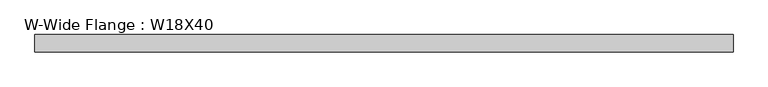
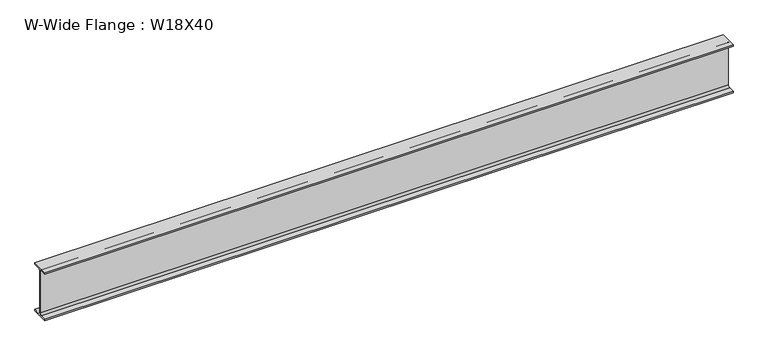
"""IFC4 building model written with IfcOpenShell, lengths in millimetres: beam geometry, W-Wide Flange : W18X40."""

from ifc_helpers import new_model, si_unit, point, frame, frame_2d, origin, place, context, project, spatial, polyline, circle_curve, trimmed, segment, composite_curve, outline, extrude, source, transform, mapped, element, save


def w_wide_flange_w18x40_5b02e5c9(model_context):
    return source(origin(), model_context, "Body", "SweptSolid", [
        extrude(outline(composite_curve([segment(polyline([(76.454, -213.995), (76.454, -227.33), (-76.454, -227.33), (-76.454, -213.995), (-20.828, -213.995)]), True, "CONTINUOUS"), segment(trimmed(circle_curve(frame_2d((-20.828, -197.1675)), 16.8275), [point((-20.828, -213.995))], [point((-4.0005, -197.1675))], True, "CARTESIAN"), True, "CONTINUOUS"), segment(polyline([(-4.0005, -197.1675), (-4.0005, 197.1675)]), True, "CONTINUOUS"), segment(trimmed(circle_curve(frame_2d((-20.828, 197.1675)), 16.8275), [point((-4.0005, 197.1675))], [point((-20.828, 213.995))], True, "CARTESIAN"), True, "CONTINUOUS"), segment(polyline([(-20.828, 213.995), (-76.454, 213.995), (-76.454, 227.33), (76.454, 227.33), (76.454, 213.995), (20.828, 213.995)]), True, "CONTINUOUS"), segment(trimmed(circle_curve(frame_2d((20.828, 197.1675)), 16.8275), [point((20.828, 213.995))], [point((4.0005, 197.1675))], True, "CARTESIAN"), True, "CONTINUOUS"), segment(polyline([(4.0005, 197.1675), (4.0005, -197.1675)]), True, "CONTINUOUS"), segment(trimmed(circle_curve(frame_2d((20.828, -197.1675)), 16.8275), [point((4.0005, -197.1675))], [point((20.828, -213.995))], True, "CARTESIAN"), True, "CONTINUOUS"), segment(polyline([(20.828, -213.995), (76.454, -213.995)]), True, "CONTINUOUS")], self_intersect=False)), frame((-3079.75, 0.0, 0.0), z_axis=(1.0, 0.0, 0.0), x_axis=(0.0, 1.0, 0.0)), (0.0, 0.0, 1.0), 6159.5),
    ])


if __name__ == "__main__":
    model = new_model("IFC4")
    model_context = context("Model", 3, world=origin())
    ifc_project = project(units=[si_unit("LENGTHUNIT", "METRE", prefix="MILLI")], contexts=[model_context])
    site = spatial("IfcSite", under=ifc_project)
    building = spatial("IfcBuilding", under=site)
    placement = place(None, origin())
    w_wide_flange_w18x40_shape = w_wide_flange_w18x40_5b02e5c9(model_context)
    element("IfcBeam", 1, ObjectType="W-Wide Flange : W18X40", at=placement, inside=building, context=model_context, shape_type="MappedRepresentation", body=[
        mapped(w_wide_flange_w18x40_shape, transform((0.0, 0.0, 0.0), x_axis=(1.0, 0.0, 0.0), y_axis=(0.0, 1.0, 0.0), z_axis=(0.0, 0.0, 1.0))),
    ])
    save(model, "model.ifc")

# Revit data of these elements
# Type "W-Wide Flange : W18X40"
#   Assembly Code = "B10"
#   W = 40
#   Length [instance default] = 5' - 0"
#   bf = 0' - 6.02"
#   d = 1' - 5.9"
#   k = 0' - 1 3/16"
#   k2 = 0' - 0.6625"
#   tf = 0' - 0.525"
#   tw = 0' - 0.315"
#   A = 0.0819444 SF
#   Structural Material [instance default] = Steel ASTM A992
# Element 1 (IfcBeam, "W-Wide Flange : W18X40")
#   Materials on its faces: "Steel ASTM A992"
# Materials
#   "Steel ASTM A992": class "Metal", colour RGB 199 199 199, transparency 0, Description = "Structural steel 50ksi", Cost = 0
